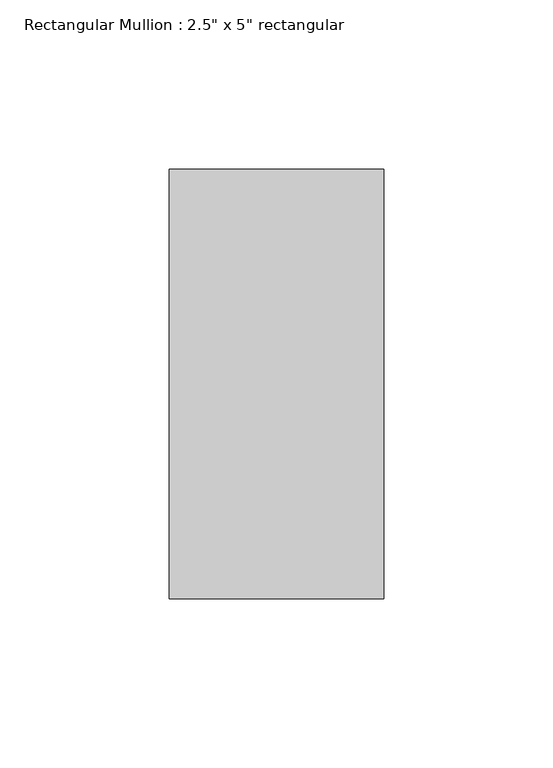
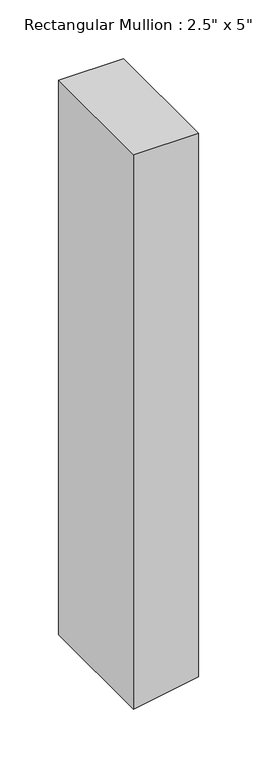
"""IFC4 building model written with IfcOpenShell, lengths in millimetres: member geometry."""

from ifc_helpers import new_model, si_unit, frame, origin, place, context, project, spatial, polyline, outline, extrude, source, transform, mapped, element, save


def member_f032fc72(model_context):
    return source(origin(), model_context, "Body", "SweptSolid", [
        extrude(outline(polyline([(0.0, 31.75), (0.0, -31.75), (-574.4884442, -31.75), (-570.8343601, -11.0266593), (-563.2916809, 31.75), (0.0, 31.75)])), frame((0.0, -63.5, 0.0), z_axis=(0.0, 1.0, 0.0), x_axis=(0.0, 0.0, 1.0)), (0.0, 0.0, 1.0), 127.0),
    ])


if __name__ == "__main__":
    model = new_model("IFC4")
    model_context = context("Model", 3, world=origin())
    ifc_project = project(units=[si_unit("LENGTHUNIT", "METRE", prefix="MILLI")], contexts=[model_context])
    site = spatial("IfcSite", under=ifc_project)
    building = spatial("IfcBuilding", under=site)
    placement = place(None, origin())
    member_shape = member_f032fc72(model_context)
    element("IfcMember", 1, ObjectType="Rectangular Mullion : 2.5\" x 5\" rectangular", at=placement, inside=building, context=model_context, shape_type="MappedRepresentation", body=[
        mapped(member_shape, transform((0.0, 0.0, 0.0), x_axis=(1.0, 0.0, 0.0), y_axis=(0.0, 1.0, 0.0), z_axis=(0.0, 0.0, 1.0))),
    ])
    save(model, "model.ifc")

# Revit data of these elements
# Type "Rectangular Mullion : 2.5\" x 5\" rectangular"
#   built-in parameter 1007304 = 0.416667 (stored number, unit not read)
#   built-in parameter 1007301 = 0.104167 (stored number, unit not read)
#   built-in parameter 1007300 = 0.104167 (stored number, unit not read)
# Element 1 (IfcMember, "Rectangular Mullion : 2.5\" x 5\" rectangular")
#   Materials on its faces: "Black Mullions"
# Materials
#   "Black Mullions": class "Wood", colour RGB 0 0 0, transparency 0, Cost = 0
